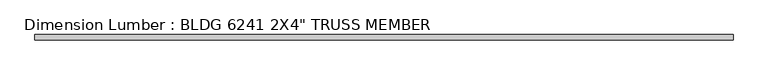
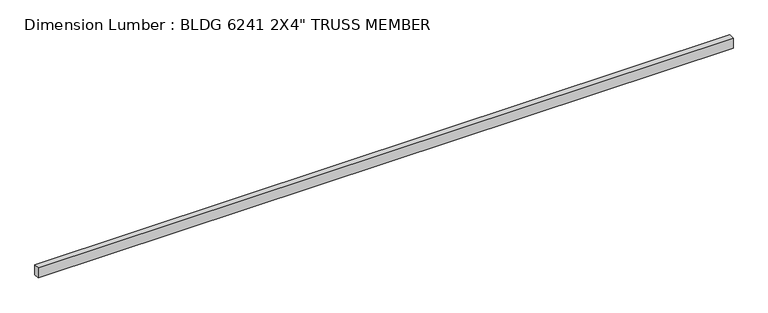
"""IFC4 building model written with IfcOpenShell, lengths in millimetres: beam geometry."""

import ifcopenshell
import ifcopenshell.guid

model = None  # the IFC model being written
_history = None  # IfcOwnerHistory: only IFC2X3 demands one
_inside = {}  # id of a spatial element -> (the spatial element, [elements in it])
_under = {}  # id of a project, library or spatial element -> (it, [spatial elements below it])
_declared = {}  # id of a project -> (the project, [libraries it declares])
_typed = {}  # id of a type object -> (the type object, [elements of that type])
_made_of = {}  # id of a material, layer set ... -> (it, [elements and type objects made of it])


def new_model(schema):
    """Start an empty IFC model of exactly this schema.

    Asked for "IFC4X3", IfcOpenShell would pick the latest addendum, in which some entities
    have other attributes; the version numbers below select the first issue.
    IFC2X3 requires an IfcOwnerHistory on every rooted entity: one is made here for all.
    """
    global model, _history
    if schema == "IFC4X3":
        model = ifcopenshell.file(schema_version=(4, 3, 0, 0))
    else:
        model = ifcopenshell.file(schema=schema)
    _inside.clear()
    _under.clear()
    _declared.clear()
    _typed.clear()
    _made_of.clear()
    _history = None
    if model.schema == "IFC2X3":
        org = make("IfcOrganization", Name="unknown")
        user = make(
            "IfcPersonAndOrganization",
            ThePerson=make("IfcPerson", FamilyName="unknown"),
            TheOrganization=org,
        )
        app = make(
            "IfcApplication",
            ApplicationDeveloper=org,
            Version="unknown",
            ApplicationFullName="unknown",
            ApplicationIdentifier="unknown",
        )
        _history = make(
            "IfcOwnerHistory",
            OwningUser=user,
            OwningApplication=app,
            ChangeAction="ADDED",
            CreationDate=0,
        )
    return model


def make(cls, **values):
    """One entity of the class cls with the attributes given. An attribute that is None is left unset."""
    return model.create_entity(
        cls, **{name: value for name, value in values.items() if value is not None}
    )


def rooted(cls, **values):
    """An entity with a GlobalId (a new one), such as an element, a storey or a relation."""
    return make(cls, GlobalId=ifcopenshell.guid.new(), OwnerHistory=_history, **values)


def si_unit(unit_type, name, prefix=None):
    """IfcSIUnit, for example si_unit("LENGTHUNIT", "METRE", prefix="MILLI")."""
    return make("IfcSIUnit", UnitType=unit_type, Prefix=prefix, Name=name)


def assignment(units):
    """IfcUnitAssignment: the units of a project."""
    return None if units is None else make("IfcUnitAssignment", Units=units)


def point(xyz):
    """IfcCartesianPoint."""
    return None if xyz is None else make("IfcCartesianPoint", Coordinates=xyz)


def direction(xyz):
    """IfcDirection."""
    return None if xyz is None else make("IfcDirection", DirectionRatios=xyz)


def frame(location, z_axis=None, x_axis=None):
    """IfcAxis2Placement3D, a coordinate frame: its origin and axes. An axis left out is left unset."""
    return make(
        "IfcAxis2Placement3D",
        Location=point(location),
        Axis=direction(z_axis),
        RefDirection=direction(x_axis),
    )


def origin():
    """The frame at (0, 0, 0) with its axes left unset."""
    return frame((0.0, 0.0, 0.0))


def place(relative_to, where):
    """IfcLocalPlacement: puts the frame where relative to a parent placement (None: the world)."""
    return make(
        "IfcLocalPlacement", PlacementRelTo=relative_to, RelativePlacement=where
    )


def context(
    kind, dimensions, precision=None, world=None, true_north=None, identifier=None
):
    """IfcGeometricRepresentationContext, for example the 3D "Model" context."""
    return make(
        "IfcGeometricRepresentationContext",
        ContextIdentifier=identifier,
        ContextType=kind,
        CoordinateSpaceDimension=dimensions,
        Precision=precision,
        WorldCoordinateSystem=world,
        TrueNorth=true_north,
    )


def project(units=None, contexts=None):
    """IfcProject with its units and contexts."""
    return rooted(
        "IfcProject",
        Name="project",
        RepresentationContexts=contexts,
        UnitsInContext=assignment(units),
    )


def spatial(cls, under=None, at=None, **own):
    """A site, building, storey or space (cls), placed at a placement, below another one or the project."""
    s = rooted(cls, ObjectPlacement=at, **own)
    if under is not None:
        _under.setdefault(under.id(), (under, []))[1].append(s)
    return s


def polyline(points):
    """IfcPolyline through the points."""
    return make("IfcPolyline", Points=[point(p) for p in points])


def outline(outer, holes=None, kind="AREA"):
    """IfcArbitraryClosedProfileDef: a profile drawn as a closed curve; with holes, ...WithVoids."""
    if holes is None:
        return make("IfcArbitraryClosedProfileDef", ProfileType=kind, OuterCurve=outer)
    return make(
        "IfcArbitraryProfileDefWithVoids",
        ProfileType=kind,
        OuterCurve=outer,
        InnerCurves=holes,
    )


def extrude(swept, where, along, depth):
    """IfcExtrudedAreaSolid: the profile swept, set in the frame where, extruded along a direction by depth."""
    return make(
        "IfcExtrudedAreaSolid",
        SweptArea=swept,
        Position=where,
        ExtrudedDirection=direction(along),
        Depth=depth,
    )


def shape(context_of_items, identifier, shape_type, items):
    """IfcShapeRepresentation: the items that make up one representation, for example the "Body"."""
    return make(
        "IfcShapeRepresentation",
        ContextOfItems=context_of_items,
        RepresentationIdentifier=identifier,
        RepresentationType=shape_type,
        Items=items,
    )


def source(mapping_origin, context_of_items, identifier, shape_type, items):
    """IfcRepresentationMap: a shape defined once, which mapped items show again and again."""
    return make(
        "IfcRepresentationMap",
        MappingOrigin=mapping_origin,
        MappedRepresentation=shape(context_of_items, identifier, shape_type, items),
    )


def transform(
    local_origin,
    x_axis=None,
    y_axis=None,
    z_axis=None,
    scale=None,
    scale2=None,
    scale3=None,
    uniform=True,
):
    """IfcCartesianTransformationOperator3D, or its non-uniform kind. x_axis, y_axis, z_axis: its Axis1, 2, 3."""
    if uniform:
        return make(
            "IfcCartesianTransformationOperator3D",
            Axis1=direction(x_axis),
            Axis2=direction(y_axis),
            LocalOrigin=point(local_origin),
            Scale=scale,
            Axis3=direction(z_axis),
        )
    return make(
        "IfcCartesianTransformationOperator3DnonUniform",
        Axis1=direction(x_axis),
        Axis2=direction(y_axis),
        LocalOrigin=point(local_origin),
        Scale=scale,
        Axis3=direction(z_axis),
        Scale2=scale2,
        Scale3=scale3,
    )


def mapped(mapping_source, mapping_target):
    """IfcMappedItem: shows the shape of a source again, moved by a transform."""
    return make(
        "IfcMappedItem", MappingSource=mapping_source, MappingTarget=mapping_target
    )


def made_of(thing, what):
    """Note that an element or type object is made of a material, layer set ...; save() writes the relation."""
    if what is not None:
        _made_of.setdefault(what.id(), (what, []))[1].append(thing)
    return thing


def element(
    cls,
    number,
    at=None,
    inside=None,
    cuts=None,
    type_object=None,
    material=None,
    context=None,
    identifier="Body",
    shape_type=None,
    held_by="IfcProductDefinitionShape",
    body=None,
    shapes=None,
    **own,
):
    """One element of the class cls, such as IfcWall. Its Tag is "e" and its number.

    at: its placement. inside: the storey or other place that contains it. cuts: it is an
    opening in that element (IfcRelVoidsElement). A single representation is given by context,
    identifier, shape_type and body (its items); several are given by shapes. held_by: the class
    of the entity that holds the representations. save() writes the other relations.
    """
    e = rooted(cls, Tag="e%d" % number, ObjectPlacement=at, **own)
    if body is not None:
        shapes = [shape(context, identifier, shape_type, body)]
    if shapes is not None:
        e.Representation = make(held_by, Representations=shapes)
    if inside is not None:
        _inside.setdefault(inside.id(), (inside, []))[1].append(e)
    if cuts is not None:
        rooted(
            "IfcRelVoidsElement", RelatingBuildingElement=cuts, RelatedOpeningElement=e
        )
    if type_object is not None:
        _typed.setdefault(type_object.id(), (type_object, []))[1].append(e)
    return made_of(e, material)


def aggregate(whole, parts):
    """IfcRelAggregates: a whole, such as a stair, and the parts it consists of."""
    return rooted("IfcRelAggregates", RelatingObject=whole, RelatedObjects=parts)


def save(model, path):
    """Write the relations noted so far, then the file.

    IfcRelAggregates (storeys below a building ...), IfcRelContainedInSpatialStructure (elements
    in a storey), IfcRelDefinesByType, IfcRelAssociatesMaterial and IfcRelDeclares: one each for
    every whole, place, type object, material and project.
    """
    for whole, parts in _under.values():
        aggregate(whole, parts)
    for where, things in _inside.values():
        rooted(
            "IfcRelContainedInSpatialStructure",
            RelatedElements=things,
            RelatingStructure=where,
        )
    for kind, things in _typed.values():
        rooted("IfcRelDefinesByType", RelatedObjects=things, RelatingType=kind)
    for what, things in _made_of.values():
        rooted("IfcRelAssociatesMaterial", RelatedObjects=things, RelatingMaterial=what)
    for by, libraries in _declared.values():
        rooted("IfcRelDeclares", RelatingContext=by, RelatedDefinitions=libraries)
    model.write(path)


def beam_4ff5e491(model_context):
    return source(origin(), model_context, "Body", "SweptSolid", [
        extrude(outline(polyline([(3248.0249994, 25.4), (3248.0249994, -25.4), (-3248.0249994, -25.4), (-3248.0249994, 25.4), (3248.0249994, 25.4)])), frame((0.0, 0.0, -50.8), z_axis=(0.0, 0.0, 1.0), x_axis=(1.0, 0.0, 0.0)), (0.0, 0.0, 1.0), 101.6),
    ])


if __name__ == "__main__":
    model = new_model("IFC4")
    model_context = context("Model", 3, world=origin())
    ifc_project = project(units=[si_unit("LENGTHUNIT", "METRE", prefix="MILLI")], contexts=[model_context])
    site = spatial("IfcSite", under=ifc_project)
    building = spatial("IfcBuilding", under=site)
    placement = place(None, origin())
    beam_shape = beam_4ff5e491(model_context)
    element("IfcBeam", 1, ObjectType="Dimension Lumber : BLDG 6241 2X4\" TRUSS MEMBER", at=placement, inside=building, context=model_context, shape_type="MappedRepresentation", body=[
        mapped(beam_shape, transform((0.0, 0.0, 0.0), x_axis=(1.0, 0.0, 0.0), y_axis=(0.0, 1.0, 0.0), z_axis=(0.0, 0.0, 1.0))),
    ])
    save(model, "model.ifc")

# Revit data of these elements
# Type "Dimension Lumber : BLDG 6241 2X4\" TRUSS MEMBER"
#   Assembly Code = "B10"
#   A = 0.273472 SF
#   Length [instance default] = 5' - 0"
#   b = 0' - 2"
#   d = 0' - 4"
#   Structural Material [instance default] = Softwood, Lumber
# Element 1 (IfcBeam, "Dimension Lumber : BLDG 6241 2X4\" TRUSS MEMBER")
#   Materials on its faces: "Softwood, Lumber"
# Materials
#   "Softwood, Lumber": class "Wood", colour RGB 223 192 134, transparency 0, Description = "Pinus Echinata", Cost = 0
